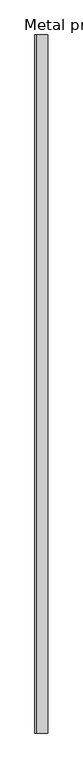
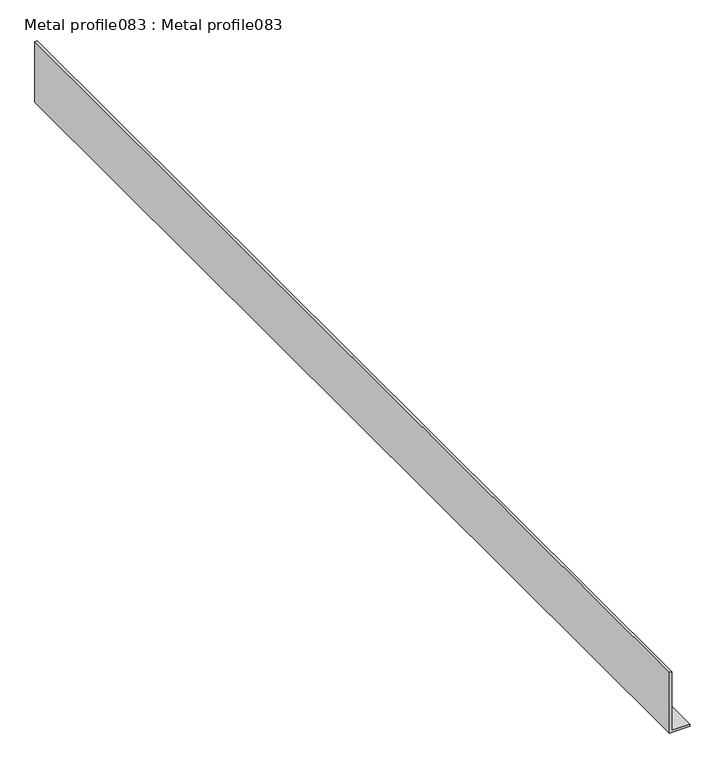
"""IFC4 building model written with IfcOpenShell, lengths in millimetres: proxy geometry, Metal profile083 : Metal profile083."""

from ifc_helpers import new_model, si_unit, frame, origin, place, context, project, spatial, polyline, outline, extrude, source, transform, mapped, element, save


def metal_profile083_metal_profile083_e6b18107(model_context):
    return source(origin(), model_context, "Body", "SweptSolid", [
        extrude(outline(polyline([(40147.8862609, -7053.4698688), (40147.8862609, -7086.4361774), (40260.5425109, -7086.4361774), (40260.5425109, -7090.4361774), (40143.8862609, -7090.4361774), (40143.8862609, -7053.4698688), (40147.8862609, -7053.4698688)])), frame((0.0, 7982.1531721, 0.0), z_axis=(0.0, 1.0, 0.0), x_axis=(0.0, 0.0, 1.0)), (0.0, 0.0, 1.0), 2000.0),
    ])


if __name__ == "__main__":
    model = new_model("IFC4")
    model_context = context("Model", 3, world=origin())
    ifc_project = project(units=[si_unit("LENGTHUNIT", "METRE", prefix="MILLI")], contexts=[model_context])
    site = spatial("IfcSite", under=ifc_project)
    building = spatial("IfcBuilding", under=site)
    placement = place(None, origin())
    metal_profile083_metal_profile083_shape = metal_profile083_metal_profile083_e6b18107(model_context)
    element("IfcBuildingElementProxy", 1, Name="Metal profile083 : Metal profile083", ObjectType="Metal profile083 : Metal profile083", at=placement, inside=building, context=model_context, shape_type="MappedRepresentation", body=[
        mapped(metal_profile083_metal_profile083_shape, transform((0.0, 0.0, 0.0), x_axis=(1.0, 0.0, 0.0), y_axis=(0.0, 1.0, 0.0), z_axis=(0.0, 0.0, 1.0))),
    ])
    save(model, "model.ifc")

# Revit data of these elements
# Type "Metal profile083 : Metal profile083"
#   NameOverride = "Metal profile083"
# Element 1 (IfcBuildingElementProxy, "Metal profile083 : Metal profile083")
#   Materials on its faces: "FIXATION SYSTEM FOR GLASS RAILING AS NEEDED"
# Materials
#   "FIXATION SYSTEM FOR GLASS RAILING AS NEEDED": class "Unassigned", colour RGB 128 128 128, transparency 0
